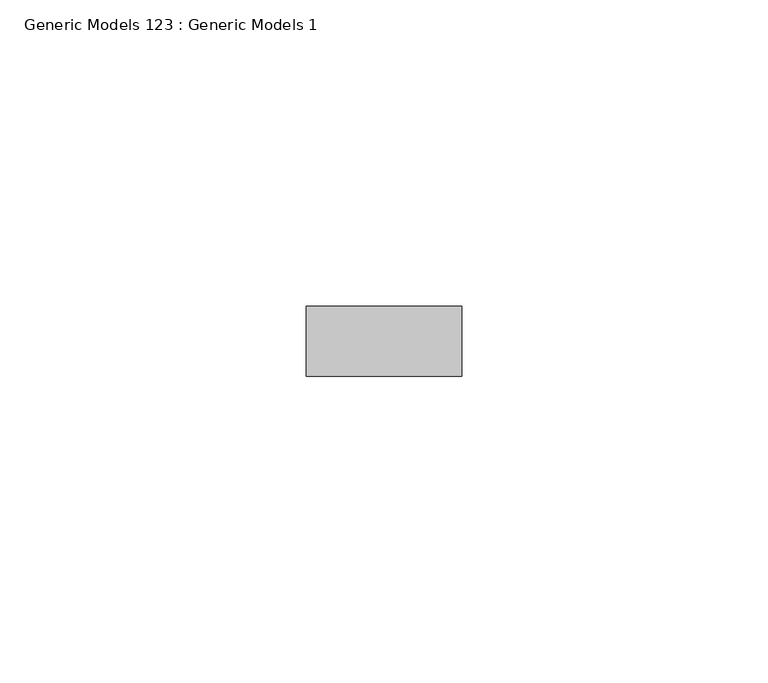
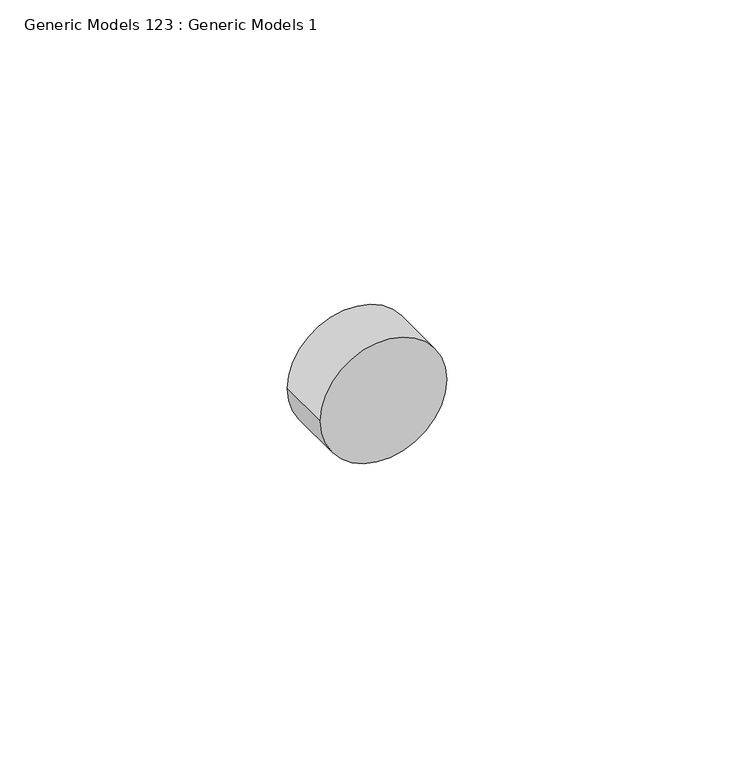
"""IFC4 building model written with IfcOpenShell, lengths in millimetres: proxy geometry, Generic Models 123 : Generic Models 1."""

from ifc_helpers import new_model, si_unit, point, frame, frame_2d, origin, place, context, project, spatial, circle_curve, trimmed, segment, composite_curve, outline, extrude, source, transform, mapped, element, save


def generic_models_123_generic_models_1_69c7d9c8(model_context):
    return source(origin(), model_context, "Body", "SweptSolid", [
        extrude(outline(composite_curve([segment(trimmed(circle_curve(frame_2d((38203.4419837, 7297.5346014)), 12.7), [point((38203.4419837, 7310.2346014))], [point((38203.4419837, 7284.8346014))], False, "CARTESIAN"), True, "CONTINUOUS"), segment(trimmed(circle_curve(frame_2d((38203.4419837, 7297.5346014)), 12.7), [point((38203.4419837, 7284.8346014))], [point((38203.4419837, 7310.2346014))], False, "CARTESIAN"), True, "CONTINUOUS")], self_intersect=False)), frame((0.0, 1836.9202358, 0.0), z_axis=(0.0, 1.0, 0.0), x_axis=(0.0, 0.0, 1.0)), (0.0, 0.0, 1.0), 11.4464372),
    ])


if __name__ == "__main__":
    model = new_model("IFC4")
    model_context = context("Model", 3, world=origin())
    ifc_project = project(units=[si_unit("LENGTHUNIT", "METRE", prefix="MILLI")], contexts=[model_context])
    site = spatial("IfcSite", under=ifc_project)
    building = spatial("IfcBuilding", under=site)
    placement = place(None, origin())
    generic_models_123_generic_models_1_shape = generic_models_123_generic_models_1_69c7d9c8(model_context)
    element("IfcBuildingElementProxy", 1, Name="Generic Models 123 : Generic Models 1", ObjectType="Generic Models 123 : Generic Models 1", at=placement, inside=building, context=model_context, shape_type="MappedRepresentation", body=[
        mapped(generic_models_123_generic_models_1_shape, transform((0.0, 0.0, 0.0), x_axis=(1.0, 0.0, 0.0), y_axis=(0.0, 1.0, 0.0), z_axis=(0.0, 0.0, 1.0))),
    ])
    save(model, "model.ifc")

# Revit data of these elements
# Element 1 (IfcBuildingElementProxy, "Generic Models 123 : Generic Models 1")
#   Materials on its faces: "S.S. LAG BOLT - SEE STRUCT. DWGS"
# Materials
#   "S.S. LAG BOLT - SEE STRUCT. DWGS": class "Generic", colour RGB 120 120 120, transparency 0, Cost = 0
